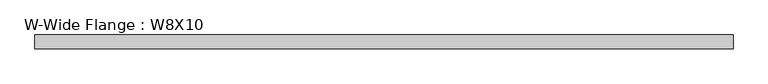
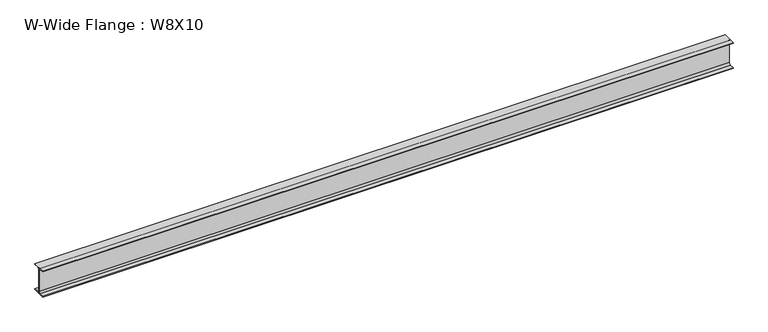
"""IFC4 building model written with IfcOpenShell, lengths in millimetres: beam geometry, W-Wide Flange : W8X10."""

from ifc_helpers import new_model, si_unit, point, frame, frame_2d, origin, place, context, project, spatial, polyline, circle_curve, trimmed, segment, composite_curve, outline, extrude, source, transform, mapped, element, save


def w_wide_flange_w8x10_45ce977e(model_context):
    return source(origin(), model_context, "Body", "SweptSolid", [
        extrude(outline(composite_curve([segment(polyline([(50.038, -94.996), (50.038, -100.203), (-50.038, -100.203), (-50.038, -94.996), (-14.4145, -94.996)]), True, "CONTINUOUS"), segment(trimmed(circle_curve(frame_2d((-14.4145, -82.7405)), 12.2555), [point((-14.4145, -94.996))], [point((-2.159, -82.7405))], True, "CARTESIAN"), True, "CONTINUOUS"), segment(polyline([(-2.159, -82.7405), (-2.159, 82.7405)]), True, "CONTINUOUS"), segment(trimmed(circle_curve(frame_2d((-14.4145, 82.7405)), 12.2555), [point((-2.159, 82.7405))], [point((-14.4145, 94.996))], True, "CARTESIAN"), True, "CONTINUOUS"), segment(polyline([(-14.4145, 94.996), (-50.038, 94.996), (-50.038, 100.203), (50.038, 100.203), (50.038, 94.996), (14.4145, 94.996)]), True, "CONTINUOUS"), segment(trimmed(circle_curve(frame_2d((14.4145, 82.7405)), 12.2555), [point((14.4145, 94.996))], [point((2.159, 82.7405))], True, "CARTESIAN"), True, "CONTINUOUS"), segment(polyline([(2.159, 82.7405), (2.159, -82.7405)]), True, "CONTINUOUS"), segment(trimmed(circle_curve(frame_2d((14.4145, -82.7405)), 12.2555), [point((2.159, -82.7405))], [point((14.4145, -94.996))], True, "CARTESIAN"), True, "CONTINUOUS"), segment(polyline([(14.4145, -94.996), (50.038, -94.996)]), True, "CONTINUOUS")], self_intersect=False)), frame((-2541.5875, 0.0, 0.0), z_axis=(1.0, 0.0, 0.0), x_axis=(0.0, 1.0, 0.0)), (0.0, 0.0, 1.0), 5083.175),
    ])


if __name__ == "__main__":
    model = new_model("IFC4")
    model_context = context("Model", 3, world=origin())
    ifc_project = project(units=[si_unit("LENGTHUNIT", "METRE", prefix="MILLI")], contexts=[model_context])
    site = spatial("IfcSite", under=ifc_project)
    building = spatial("IfcBuilding", under=site)
    placement = place(None, origin())
    w_wide_flange_w8x10_shape = w_wide_flange_w8x10_45ce977e(model_context)
    element("IfcBeam", 1, ObjectType="W-Wide Flange : W8X10", at=placement, inside=building, context=model_context, shape_type="MappedRepresentation", body=[
        mapped(w_wide_flange_w8x10_shape, transform((0.0, 0.0, 0.0), x_axis=(1.0, 0.0, 0.0), y_axis=(0.0, 1.0, 0.0), z_axis=(0.0, 0.0, 1.0))),
    ])
    save(model, "model.ifc")

# Revit data of these elements
# Type "W-Wide Flange : W8X10"
#   Assembly Code = "B10"
#   W = 10
#   Length [instance default] = 1524 mm
#   bf = 100.076 mm
#   d = 200.406 mm
#   k = 17.463 mm
#   k2 = 12.255 mm
#   tf = 5.207 mm
#   tw = 4.318 mm
#   A = 0.00190967 m²
#   Structural Material [instance default] = Steel ASTM A992
# Element 1 (IfcBeam, "W-Wide Flange : W8X10")
#   Structural Material = Aluminum, Anodized Red
#   Materials on its faces: "Aluminum, Anodized Red"
# Materials
#   "Steel ASTM A992": class "Metal", colour RGB 128 0 0, transparency 0, Description = "Structural steel 50ksi", Cost = 0
#   "Aluminum, Anodized Red": class "Metal", colour RGB 120 120 120, transparency 0, Description = "Anodized aluminum, red", Cost = 0
